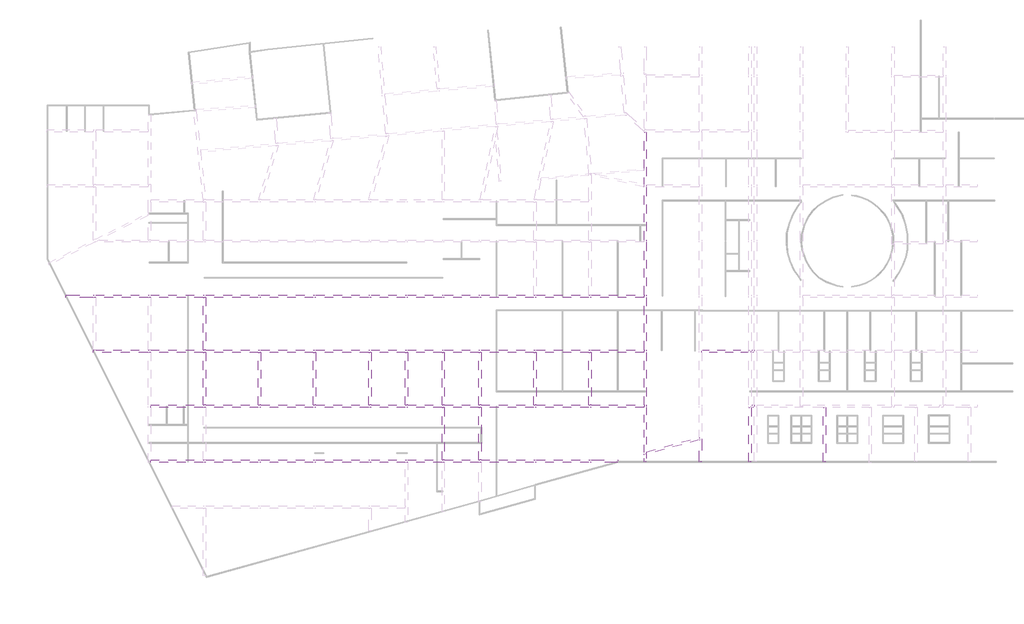
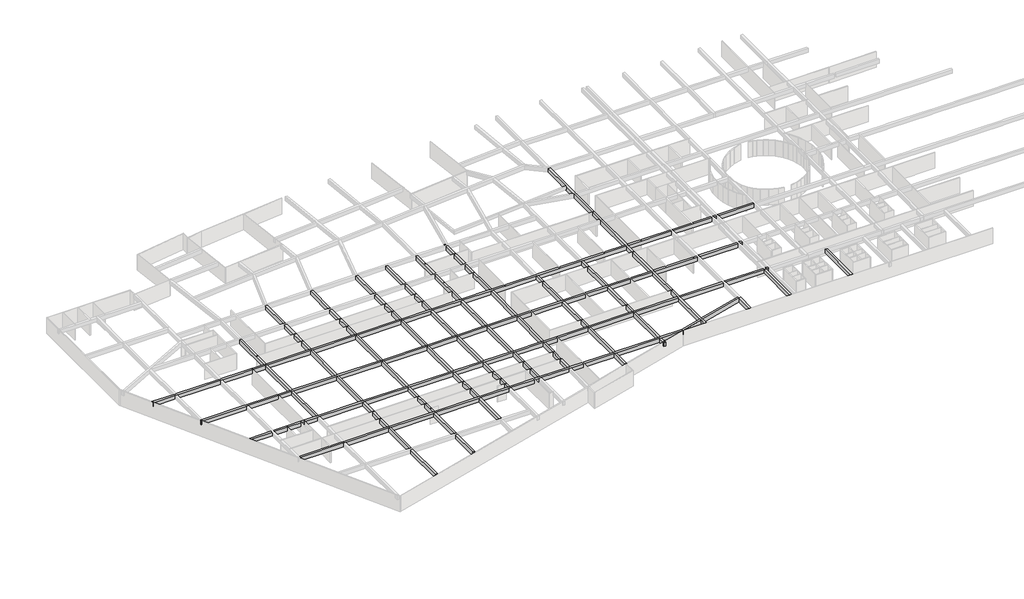
# One storey, part 5 of 8: 24 beams.
"""IFC4 building model written with IfcOpenShell, lengths in millimetres."""

from ifc_helpers import new_model, si_unit, frame, origin, place, context, project, spatial, polyline, outline, extrude, faceted_brep, element, save

model = new_model("IFC4")

# Units and contexts
model_context = context("Model", 3, world=origin())
ifc_project = project(units=[si_unit("LENGTHUNIT", "METRE", prefix="MILLI")], contexts=[model_context])

# Site, building, storey
site = spatial("IfcSite", under=ifc_project)
building = spatial("IfcBuilding", under=site)
storey = spatial("IfcBuildingStorey", under=building, Name="户型图", Elevation=0.0)

# Beams
placement = place(None, origin())
element("IfcBeam", 1, ObjectType="混凝土 - 矩形梁 : KL_beam", at=placement, inside=storey, context=model_context, shape_type="Brep", body=[
    faceted_brep([(397553.8653576, -29561.3735341, 3300.0), (397153.8653576, -29561.3735341, 3300.0), (397153.8653576, -29561.3735341, 2500.0), (397553.8653576, -29561.3735341, 2500.0), (397553.8653576, -28340.5712105, 3300.0), (397553.8653576, -27925.4258396, 3300.0), (397553.8653576, -20661.3735124, 3300.0), (397553.8653576, -20261.3735124, 3300.0), (397553.8653576, -11661.3735096, 3300.0), (397553.8653576, -11261.3735096, 3300.0), (397553.8653576, -2661.3735096, 3300.0), (397553.8653576, -2261.3735096, 3300.0), (397553.8653576, 6338.6264904, 3300.0), (397553.8653576, 6738.6264904, 3300.0), (397553.8653576, 15338.6264904, 3300.0), (397553.8653576, 15738.6264904, 3300.0), (397553.8653576, 24338.6264659, 3300.0), (397153.8653576, 24338.6264659, 3300.0), (397153.8653576, 18348.9010914, 3300.0), (397153.8653576, 18047.7660466, 3300.0), (397153.8653576, 15787.9497009, 3300.0), (397153.8653576, 15378.1921694, 3300.0), (397153.8653576, 6738.6264904, 3300.0), (397153.8653576, 6338.6264904, 3300.0), (397153.8653576, -2261.3735096, 3300.0), (397153.8653576, -2661.3735096, 3300.0), (397153.8653576, -11261.3735096, 3300.0), (397153.8653576, -11661.3735096, 3300.0), (397153.8653576, -20261.3735124, 3300.0), (397153.8653576, -20661.3735124, 3300.0), (397153.8653576, -28036.5369507, 3300.0), (397153.8653576, -28451.6823216, 3300.0), (397153.8653576, 24338.6264659, 2500.0), (397153.8653576, 15787.9497009, 2500.0), (397153.8653576, 15378.1921694, 2500.0), (397153.8653576, 6738.6264904, 2500.0), (397153.8653576, 6338.6264904, 2500.0), (397153.8653576, -2261.3735096, 2500.0), (397153.8653576, -2661.3735096, 2500.0), (397153.8653576, -11261.3735096, 2500.0), (397153.8653576, -11661.3735096, 2500.0), (397153.8653576, -20261.3735124, 2500.0), (397153.8653576, -20661.3735124, 2500.0), (397153.8653576, -28036.5369507, 2500.0), (397153.8653576, -28451.6823216, 2500.0), (397553.8653576, 24338.6264659, 2500.0), (397553.8653576, 15738.6264904, 2500.0), (397553.8653576, 15338.6264904, 2500.0), (397553.8653576, 6738.6264904, 2500.0), (397553.8653576, 6338.6264904, 2500.0), (397553.8653576, -2261.3735096, 2500.0), (397553.8653576, -2661.3735096, 2500.0), (397553.8653576, -11261.3735096, 2500.0), (397553.8653576, -11661.3735096, 2500.0), (397553.8653576, -20261.3735124, 2500.0), (397553.8653576, -20661.3735124, 2500.0), (397553.8653576, -27925.4258396, 2500.0), (397553.8653576, -28340.5712105, 2500.0)], [[[0, 1, 2, 3]], [[1, 0, 4, 5, 6, 7, 8, 9, 10, 11, 12, 13, 14, 15, 16, 17, 18, 19, 20, 21, 22, 23, 24, 25, 26, 27, 28, 29, 30, 31]], [[2, 1, 31, 30, 29, 28, 27, 26, 25, 24, 23, 22, 21, 20, 19, 18, 17, 32, 33, 34, 35, 36, 37, 38, 39, 40, 41, 42, 43, 44]], [[3, 2, 44, 43, 42, 41, 40, 39, 38, 37, 36, 35, 34, 33, 32, 45, 46, 47, 48, 49, 50, 51, 52, 53, 54, 55, 56, 57]], [[0, 3, 57, 56, 55, 54, 53, 52, 51, 50, 49, 48, 47, 46, 45, 16, 15, 14, 13, 12, 11, 10, 9, 8, 7, 6, 5, 4]], [[17, 16, 45, 32]]]),
])
element("IfcBeam", 2, ObjectType="混凝土 - 矩形梁 : KL_beam", at=placement, inside=storey, context=model_context, shape_type="Brep", body=[
    faceted_brep([(406153.8653576, -11661.3735096, 3300.0), (406153.8653576, -11261.3735096, 3300.0), (397553.8653576, -11261.3735096, 3300.0), (397553.8653576, -11661.3735096, 3300.0), (406153.8653576, -11261.3735096, 2500.0), (397553.8653576, -11261.3735096, 2500.0), (406153.8653576, -11661.3735096, 2500.0), (397553.8653576, -11661.3735096, 2500.0)], [[[0, 1, 2, 3]], [[1, 4, 5, 2]], [[4, 6, 7, 5]], [[6, 0, 3, 7]], [[1, 0, 6, 4]], [[3, 2, 5, 7]]]),
    faceted_brep([(397153.8653576, -11261.3735096, 3300.0), (397153.8653576, -11661.3735096, 3300.0), (397153.8653576, -11661.3735096, 2500.0), (397153.8653576, -11261.3735096, 2500.0), (307153.8653555, -11261.3735096, 3300.0), (307153.8653555, -11661.3735096, 3300.0), (316153.8653576, -11661.3735096, 3300.0), (316553.8653576, -11661.3735096, 3300.0), (325153.8653576, -11661.3735096, 3300.0), (325553.8653576, -11661.3735096, 3300.0), (334153.8653576, -11661.3735096, 3300.0), (334553.8653576, -11661.3735096, 3300.0), (343153.8653576, -11661.3735096, 3300.0), (343553.8653576, -11661.3735096, 3300.0), (352153.8653576, -11661.3735096, 3300.0), (352553.8653576, -11661.3735096, 3300.0), (358153.8653576, -11661.3735096, 3300.0), (358553.8653576, -11661.3735096, 3300.0), (364153.8653576, -11661.3735096, 3300.0), (364553.8653576, -11661.3735096, 3300.0), (370153.8653576, -11661.3735096, 3300.0), (370553.8653576, -11661.3735096, 3300.0), (379153.8653576, -11661.3735096, 3300.0), (379553.8653576, -11661.3735096, 3300.0), (388153.8653576, -11661.3735096, 3300.0), (388553.8653576, -11661.3735096, 3300.0), (388553.8653576, -11261.3735096, 3300.0), (388153.8653576, -11261.3735096, 3300.0), (379553.8653576, -11261.3735096, 3300.0), (379153.8653576, -11261.3735096, 3300.0), (370553.8653576, -11261.3735096, 3300.0), (370153.8653576, -11261.3735096, 3300.0), (364553.8653576, -11261.3735096, 3300.0), (364153.8653576, -11261.3735096, 3300.0), (358553.8653576, -11261.3735096, 3300.0), (358153.8653576, -11261.3735096, 3300.0), (352553.8653576, -11261.3735096, 3300.0), (352153.8653576, -11261.3735096, 3300.0), (343553.8653576, -11261.3735096, 3300.0), (343153.8653576, -11261.3735096, 3300.0), (334553.8653576, -11261.3735096, 3300.0), (334153.8653576, -11261.3735096, 3300.0), (325553.8653576, -11261.3735096, 3300.0), (325153.8653576, -11261.3735096, 3300.0), (316553.8653576, -11261.3735096, 3300.0), (316153.8653576, -11261.3735096, 3300.0), (307553.8653555, -11261.3735096, 3300.0), (307153.8653555, -11261.3735096, 2500.0), (388553.8653576, -11261.3735096, 2500.0), (388153.8653576, -11261.3735096, 2500.0), (379553.8653576, -11261.3735096, 2500.0), (379153.8653576, -11261.3735096, 2500.0), (370553.8653576, -11261.3735096, 2500.0), (370153.8653576, -11261.3735096, 2500.0), (364553.8653576, -11261.3735096, 2500.0), (364153.8653576, -11261.3735096, 2500.0), (358553.8653576, -11261.3735096, 2500.0), (358153.8653576, -11261.3735096, 2500.0), (352553.8653576, -11261.3735096, 2500.0), (352153.8653576, -11261.3735096, 2500.0), (343553.8653576, -11261.3735096, 2500.0), (343153.8653576, -11261.3735096, 2500.0), (334553.8653576, -11261.3735096, 2500.0), (334153.8653576, -11261.3735096, 2500.0), (325553.8653576, -11261.3735096, 2500.0), (325153.8653576, -11261.3735096, 2500.0), (316553.8653576, -11261.3735096, 2500.0), (316153.8653576, -11261.3735096, 2500.0), (307553.8653555, -11261.3735096, 2500.0), (307153.8653555, -11661.3735096, 2500.0), (388553.8653576, -11661.3735096, 2500.0), (388153.8653576, -11661.3735096, 2500.0), (379553.8653576, -11661.3735096, 2500.0), (379153.8653576, -11661.3735096, 2500.0), (370553.8653576, -11661.3735096, 2500.0), (370153.8653576, -11661.3735096, 2500.0), (364553.8653576, -11661.3735096, 2500.0), (364153.8653576, -11661.3735096, 2500.0), (358553.8653576, -11661.3735096, 2500.0), (358153.8653576, -11661.3735096, 2500.0), (352553.8653576, -11661.3735096, 2500.0), (352153.8653576, -11661.3735096, 2500.0), (343553.8653576, -11661.3735096, 2500.0), (343153.8653576, -11661.3735096, 2500.0), (334553.8653576, -11661.3735096, 2500.0), (334153.8653576, -11661.3735096, 2500.0), (325553.8653576, -11661.3735096, 2500.0), (325153.8653576, -11661.3735096, 2500.0), (316553.8653576, -11661.3735096, 2500.0), (316153.8653576, -11661.3735096, 2500.0)], [[[0, 1, 2, 3]], [[4, 5, 6, 7, 8, 9, 10, 11, 12, 13, 14, 15, 16, 17, 18, 19, 20, 21, 22, 23, 24, 25, 1, 0, 26, 27, 28, 29, 30, 31, 32, 33, 34, 35, 36, 37, 38, 39, 40, 41, 42, 43, 44, 45, 46]], [[47, 4, 46, 45, 44, 43, 42, 41, 40, 39, 38, 37, 36, 35, 34, 33, 32, 31, 30, 29, 28, 27, 26, 0, 3, 48, 49, 50, 51, 52, 53, 54, 55, 56, 57, 58, 59, 60, 61, 62, 63, 64, 65, 66, 67, 68]], [[69, 47, 68, 67, 66, 65, 64, 63, 62, 61, 60, 59, 58, 57, 56, 55, 54, 53, 52, 51, 50, 49, 48, 3, 2, 70, 71, 72, 73, 74, 75, 76, 77, 78, 79, 80, 81, 82, 83, 84, 85, 86, 87, 88, 89]], [[5, 69, 89, 88, 87, 86, 85, 84, 83, 82, 81, 80, 79, 78, 77, 76, 75, 74, 73, 72, 71, 70, 2, 1, 25, 24, 23, 22, 21, 20, 19, 18, 17, 16, 15, 14, 13, 12, 11, 10, 9, 8, 7, 6]], [[5, 4, 47, 69]]]),
])
element("IfcBeam", 3, ObjectType="混凝土 - 矩形梁 : KL_beam", at=placement, inside=storey, context=model_context, shape_type="Brep", body=[
    faceted_brep([(302728.8653513, -2261.3735096, 3300.0), (302728.8653513, -2261.3735096, 2500.0), (302728.8653513, -2661.3735096, 2500.0), (302728.8653513, -2661.3735096, 3300.0), (397153.8653576, -2261.3735096, 3300.0), (397153.8653576, -2661.3735096, 3300.0), (397153.8653576, -2661.3735096, 2500.0), (397153.8653576, -2261.3735096, 2500.0), (307153.8653555, -2661.3735096, 3300.0), (307553.8653555, -2661.3735096, 3300.0), (316153.8653576, -2661.3735096, 3300.0), (316553.8653576, -2661.3735096, 3300.0), (325153.8653576, -2661.3735096, 3300.0), (325553.8653576, -2661.3735096, 3300.0), (334153.8653576, -2661.3735096, 3300.0), (334553.8653576, -2661.3735096, 3300.0), (343153.8653576, -2661.3735096, 3300.0), (343553.8653576, -2661.3735096, 3300.0), (352153.8653576, -2661.3735096, 3300.0), (352553.8653576, -2661.3735096, 3300.0), (358153.8653576, -2661.3735096, 3300.0), (358553.8653576, -2661.3735096, 3300.0), (364153.8653576, -2661.3735096, 3300.0), (364553.8653576, -2661.3735096, 3300.0), (370153.8653576, -2661.3735096, 3300.0), (370553.8653576, -2661.3735096, 3300.0), (379153.8653576, -2661.3735096, 3300.0), (379553.8653576, -2661.3735096, 3300.0), (388153.8653576, -2661.3735096, 3300.0), (388553.8653576, -2661.3735096, 3300.0), (388553.8653576, -2261.3735096, 3300.0), (388153.8653576, -2261.3735096, 3300.0), (379553.8653576, -2261.3735096, 3300.0), (379153.8653576, -2261.3735096, 3300.0), (370553.8653576, -2261.3735096, 3300.0), (370153.8653576, -2261.3735096, 3300.0), (364553.8653576, -2261.3735096, 3300.0), (364153.8653576, -2261.3735096, 3300.0), (358553.8653576, -2261.3735096, 3300.0), (358153.8653576, -2261.3735096, 3300.0), (352553.8653576, -2261.3735096, 3300.0), (352153.8653576, -2261.3735096, 3300.0), (343553.8653576, -2261.3735096, 3300.0), (343153.8653576, -2261.3735096, 3300.0), (334553.8653576, -2261.3735096, 3300.0), (334153.8653576, -2261.3735096, 3300.0), (325553.8653576, -2261.3735096, 3300.0), (325153.8653576, -2261.3735096, 3300.0), (316553.8653576, -2261.3735096, 3300.0), (316153.8653576, -2261.3735096, 3300.0), (307553.8653555, -2261.3735096, 3300.0), (307153.8653555, -2261.3735096, 3300.0), (307153.8653555, -2661.3735096, 2500.0), (307553.8653555, -2661.3735096, 2500.0), (316153.8653576, -2661.3735096, 2500.0), (316553.8653576, -2661.3735096, 2500.0), (325153.8653576, -2661.3735096, 2500.0), (325553.8653576, -2661.3735096, 2500.0), (334153.8653576, -2661.3735096, 2500.0), (334553.8653576, -2661.3735096, 2500.0), (343153.8653576, -2661.3735096, 2500.0), (343553.8653576, -2661.3735096, 2500.0), (352153.8653576, -2661.3735096, 2500.0), (352553.8653576, -2661.3735096, 2500.0), (358153.8653576, -2661.3735096, 2500.0), (358553.8653576, -2661.3735096, 2500.0), (364153.8653576, -2661.3735096, 2500.0), (364553.8653576, -2661.3735096, 2500.0), (370153.8653576, -2661.3735096, 2500.0), (370553.8653576, -2661.3735096, 2500.0), (379153.8653576, -2661.3735096, 2500.0), (379553.8653576, -2661.3735096, 2500.0), (388153.8653576, -2661.3735096, 2500.0), (388553.8653576, -2661.3735096, 2500.0), (307153.8653555, -2261.3735096, 2500.0), (307553.8653555, -2261.3735096, 2500.0), (316153.8653576, -2261.3735096, 2500.0), (316553.8653576, -2261.3735096, 2500.0), (325153.8653576, -2261.3735096, 2500.0), (325553.8653576, -2261.3735096, 2500.0), (334153.8653576, -2261.3735096, 2500.0), (334553.8653576, -2261.3735096, 2500.0), (343153.8653576, -2261.3735096, 2500.0), (343553.8653576, -2261.3735096, 2500.0), (352153.8653576, -2261.3735096, 2500.0), (352553.8653576, -2261.3735096, 2500.0), (358153.8653576, -2261.3735096, 2500.0), (358553.8653576, -2261.3735096, 2500.0), (364153.8653576, -2261.3735096, 2500.0), (364553.8653576, -2261.3735096, 2500.0), (370153.8653576, -2261.3735096, 2500.0), (370553.8653576, -2261.3735096, 2500.0), (379153.8653576, -2261.3735096, 2500.0), (379553.8653576, -2261.3735096, 2500.0), (388153.8653576, -2261.3735096, 2500.0), (388553.8653576, -2261.3735096, 2500.0)], [[[0, 1, 2, 3]], [[4, 5, 6, 7]], [[0, 3, 8, 9, 10, 11, 12, 13, 14, 15, 16, 17, 18, 19, 20, 21, 22, 23, 24, 25, 26, 27, 28, 29, 5, 4, 30, 31, 32, 33, 34, 35, 36, 37, 38, 39, 40, 41, 42, 43, 44, 45, 46, 47, 48, 49, 50, 51]], [[3, 2, 52, 53, 54, 55, 56, 57, 58, 59, 60, 61, 62, 63, 64, 65, 66, 67, 68, 69, 70, 71, 72, 73, 6, 5, 29, 28, 27, 26, 25, 24, 23, 22, 21, 20, 19, 18, 17, 16, 15, 14, 13, 12, 11, 10, 9, 8]], [[2, 1, 74, 75, 76, 77, 78, 79, 80, 81, 82, 83, 84, 85, 86, 87, 88, 89, 90, 91, 92, 93, 94, 95, 7, 6, 73, 72, 71, 70, 69, 68, 67, 66, 65, 64, 63, 62, 61, 60, 59, 58, 57, 56, 55, 54, 53, 52]], [[1, 0, 51, 50, 49, 48, 47, 46, 45, 44, 43, 42, 41, 40, 39, 38, 37, 36, 35, 34, 33, 32, 31, 30, 4, 7, 95, 94, 93, 92, 91, 90, 89, 88, 87, 86, 85, 84, 83, 82, 81, 80, 79, 78, 77, 76, 75, 74]]]),
    faceted_brep([(422653.8653576, -2661.3735096, 3300.0), (422653.8653576, -2261.3735096, 3300.0), (415553.8653576, -2261.3735096, 3300.0), (415553.8653576, -2661.3735096, 3300.0), (422653.8653576, -2661.3735096, 2500.0), (415553.8653576, -2661.3735096, 2500.0), (422653.8653576, -2261.3735096, 2500.0), (415553.8653576, -2261.3735096, 2500.0)], [[[0, 1, 2, 3]], [[4, 0, 3, 5]], [[6, 4, 5, 7]], [[1, 6, 7, 2]], [[1, 0, 4, 6]], [[3, 2, 7, 5]]]),
    faceted_brep([(415153.8653576, -2261.3735096, 3300.0), (415153.8653576, -2661.3735096, 3300.0), (415153.8653576, -2661.3735096, 2500.0), (415153.8653576, -2261.3735096, 2500.0), (414653.8653576, -2261.3735096, 3300.0), (414653.8653576, -2661.3735096, 3300.0), (414653.8653576, -2661.3735096, 2500.0), (414653.8653576, -2261.3735096, 2500.0)], [[[0, 1, 2, 3]], [[1, 0, 4, 5]], [[2, 1, 5, 6]], [[3, 2, 6, 7]], [[0, 3, 7, 4]], [[5, 4, 7, 6]]]),
    faceted_brep([(414253.8653576, -2261.3735096, 3300.0), (414253.8653576, -2661.3735096, 3300.0), (414253.8653576, -2661.3735096, 2500.0), (414253.8653576, -2261.3735096, 2500.0), (406553.8653576, -2261.3735096, 3300.0), (406553.8653576, -2661.3735096, 3300.0), (406553.8653576, -2661.3735096, 2500.0), (406553.8653576, -2261.3735096, 2500.0)], [[[0, 1, 2, 3]], [[1, 0, 4, 5]], [[2, 1, 5, 6]], [[3, 2, 6, 7]], [[0, 3, 7, 4]], [[5, 4, 7, 6]]]),
    faceted_brep([(406153.8653576, -2261.3735096, 3300.0), (406153.8653576, -2661.3735096, 3300.0), (406153.8653576, -2661.3735096, 2500.0), (406153.8653576, -2261.3735096, 2500.0), (397553.8653576, -2261.3735096, 3300.0), (397553.8653576, -2661.3735096, 3300.0), (397553.8653576, -2661.3735096, 2500.0), (397553.8653576, -2261.3735096, 2500.0)], [[[0, 1, 2, 3]], [[1, 0, 4, 5]], [[2, 1, 5, 6]], [[3, 2, 6, 7]], [[0, 3, 7, 4]], [[5, 4, 7, 6]]]),
])
element("IfcBeam", 4, ObjectType="混凝土 - 矩形梁 : KL_beam", at=placement, inside=storey, context=model_context, shape_type="SweptSolid", body=[
    extrude(outline(polyline([(325153.8653576, 6338.6264904), (325553.8653576, 6338.6264904), (325553.8653576, -2261.3735096), (325153.8653576, -2261.3735096), (325153.8653576, 6338.6264904)])), frame((0.0, 0.0, 2500.0), z_axis=(0.0, 0.0, 1.0), x_axis=(1.0, 0.0, 0.0)), (0.0, 0.0, 1.0), 800.0),
    extrude(outline(polyline([(325553.8653576, -11261.3735096), (325153.8653576, -11261.3735096), (325153.8653576, -2661.3735096), (325553.8653576, -2661.3735096), (325553.8653576, -11261.3735096)])), frame((0.0, 0.0, 2500.0), z_axis=(0.0, 0.0, 1.0), x_axis=(1.0, 0.0, 0.0)), (0.0, 0.0, 1.0), 800.0),
])
element("IfcBeam", 5, ObjectType="混凝土 - 矩形梁 : KL_beam", at=placement, inside=storey, context=model_context, shape_type="Brep", body=[
    faceted_brep([(311853.8653587, -20261.3735124, 3300.0), (311853.8653587, -20261.3735124, 2500.0), (311853.8653587, -20661.3735124, 2500.0), (311853.8653587, -20661.3735124, 3300.0), (316153.8653576, -20261.3735124, 3300.0), (316153.8653576, -20661.3735124, 3300.0), (316153.8653576, -20661.3735124, 2500.0), (316153.8653576, -20261.3735124, 2500.0)], [[[0, 1, 2, 3]], [[4, 5, 6, 7]], [[0, 3, 5, 4]], [[3, 2, 6, 5]], [[2, 1, 7, 6]], [[1, 0, 4, 7]]]),
    faceted_brep([(414253.8653576, -20661.3735124, 3300.0), (414253.8653576, -20261.3735124, 3300.0), (406553.8653576, -20261.3735124, 3300.0), (406553.8653576, -20661.3735124, 3300.0), (414253.8653576, -20661.3735124, 2500.0), (406553.8653576, -20661.3735124, 2500.0), (414253.8653576, -20261.3735124, 2500.0), (406553.8653576, -20261.3735124, 2500.0)], [[[0, 1, 2, 3]], [[4, 0, 3, 5]], [[6, 4, 5, 7]], [[1, 6, 7, 2]], [[1, 0, 4, 6]], [[3, 2, 7, 5]]]),
    faceted_brep([(406153.8653576, -20261.3735124, 3300.0), (406153.8653576, -20661.3735124, 3300.0), (406153.8653576, -20661.3735124, 2500.0), (406153.8653576, -20261.3735124, 2500.0), (397553.8653576, -20261.3735124, 3300.0), (397553.8653576, -20661.3735124, 3300.0), (397553.8653576, -20661.3735124, 2500.0), (397553.8653576, -20261.3735124, 2500.0)], [[[0, 1, 2, 3]], [[1, 0, 4, 5]], [[2, 1, 5, 6]], [[3, 2, 6, 7]], [[0, 3, 7, 4]], [[5, 4, 7, 6]]]),
    faceted_brep([(397153.8653576, -20261.3735124, 3300.0), (397153.8653576, -20661.3735124, 3300.0), (397153.8653576, -20661.3735124, 2500.0), (397153.8653576, -20261.3735124, 2500.0), (388553.8653576, -20261.3735124, 3300.0), (388153.8653576, -20261.3735124, 3300.0), (379553.8653576, -20261.3735124, 3300.0), (379153.8653576, -20261.3735124, 3300.0), (370553.8653576, -20261.3735124, 3300.0), (370153.8653576, -20261.3735124, 3300.0), (364553.8653576, -20261.3735124, 3300.0), (364153.8653576, -20261.3735124, 3300.0), (358553.8653576, -20261.3735124, 3300.0), (358153.8653576, -20261.3735124, 3300.0), (352553.8653576, -20261.3735124, 3300.0), (352153.8653576, -20261.3735124, 3300.0), (343553.8653576, -20261.3735124, 3300.0), (343153.8653576, -20261.3735124, 3300.0), (334553.8653576, -20261.3735124, 3300.0), (334153.8653576, -20261.3735124, 3300.0), (325553.8653576, -20261.3735124, 3300.0), (325153.8653576, -20261.3735124, 3300.0), (316553.8653576, -20261.3735124, 3300.0), (316553.8653576, -20661.3735124, 3300.0), (325153.8653576, -20661.3735124, 3300.0), (325553.8653576, -20661.3735124, 3300.0), (334153.8653576, -20661.3735124, 3300.0), (334553.8653576, -20661.3735124, 3300.0), (343153.8653576, -20661.3735124, 3300.0), (343553.8653576, -20661.3735124, 3300.0), (352153.8653576, -20661.3735124, 3300.0), (352553.8653576, -20661.3735124, 3300.0), (358153.8653576, -20661.3735124, 3300.0), (358553.8653576, -20661.3735124, 3300.0), (364153.8653576, -20661.3735124, 3300.0), (364553.8653576, -20661.3735124, 3300.0), (370153.8653576, -20661.3735124, 3300.0), (370553.8653576, -20661.3735124, 3300.0), (379153.8653576, -20661.3735124, 3300.0), (379553.8653576, -20661.3735124, 3300.0), (388153.8653576, -20661.3735124, 3300.0), (388553.8653576, -20661.3735124, 3300.0), (316553.8653576, -20661.3735124, 2500.0), (325153.8653576, -20661.3735124, 2500.0), (325553.8653576, -20661.3735124, 2500.0), (334153.8653576, -20661.3735124, 2500.0), (334553.8653576, -20661.3735124, 2500.0), (343153.8653576, -20661.3735124, 2500.0), (343553.8653576, -20661.3735124, 2500.0), (352153.8653576, -20661.3735124, 2500.0), (352553.8653576, -20661.3735124, 2500.0), (358153.8653576, -20661.3735124, 2500.0), (358553.8653576, -20661.3735124, 2500.0), (364153.8653576, -20661.3735124, 2500.0), (364553.8653576, -20661.3735124, 2500.0), (370153.8653576, -20661.3735124, 2500.0), (370553.8653576, -20661.3735124, 2500.0), (379153.8653576, -20661.3735124, 2500.0), (379553.8653576, -20661.3735124, 2500.0), (388153.8653576, -20661.3735124, 2500.0), (388553.8653576, -20661.3735124, 2500.0), (316553.8653576, -20261.3735124, 2500.0), (325153.8653576, -20261.3735124, 2500.0), (325553.8653576, -20261.3735124, 2500.0), (334153.8653576, -20261.3735124, 2500.0), (334553.8653576, -20261.3735124, 2500.0), (343153.8653576, -20261.3735124, 2500.0), (343553.8653576, -20261.3735124, 2500.0), (352153.8653576, -20261.3735124, 2500.0), (352553.8653576, -20261.3735124, 2500.0), (358153.8653576, -20261.3735124, 2500.0), (358553.8653576, -20261.3735124, 2500.0), (364153.8653576, -20261.3735124, 2500.0), (364553.8653576, -20261.3735124, 2500.0), (370153.8653576, -20261.3735124, 2500.0), (370553.8653576, -20261.3735124, 2500.0), (379153.8653576, -20261.3735124, 2500.0), (379553.8653576, -20261.3735124, 2500.0), (388153.8653576, -20261.3735124, 2500.0), (388553.8653576, -20261.3735124, 2500.0)], [[[0, 1, 2, 3]], [[1, 0, 4, 5, 6, 7, 8, 9, 10, 11, 12, 13, 14, 15, 16, 17, 18, 19, 20, 21, 22, 23, 24, 25, 26, 27, 28, 29, 30, 31, 32, 33, 34, 35, 36, 37, 38, 39, 40, 41]], [[2, 1, 41, 40, 39, 38, 37, 36, 35, 34, 33, 32, 31, 30, 29, 28, 27, 26, 25, 24, 23, 42, 43, 44, 45, 46, 47, 48, 49, 50, 51, 52, 53, 54, 55, 56, 57, 58, 59, 60]], [[3, 2, 60, 59, 58, 57, 56, 55, 54, 53, 52, 51, 50, 49, 48, 47, 46, 45, 44, 43, 42, 61, 62, 63, 64, 65, 66, 67, 68, 69, 70, 71, 72, 73, 74, 75, 76, 77, 78, 79]], [[0, 3, 79, 78, 77, 76, 75, 74, 73, 72, 71, 70, 69, 68, 67, 66, 65, 64, 63, 62, 61, 22, 21, 20, 19, 18, 17, 16, 15, 14, 13, 12, 11, 10, 9, 8, 7, 6, 5, 4]], [[23, 22, 61, 42]]]),
])
element("IfcBeam", 6, ObjectType="混凝土 - 矩形梁 : KL_beam", at=placement, inside=storey, context=model_context, shape_type="SweptSolid", body=[
    extrude(outline(polyline([(414653.8653576, -29561.3735124), (414253.8653576, -29561.3735124), (414253.8653576, -20661.3735124), (414653.8653576, -20661.3735124), (414653.8653576, -29561.3735124)])), frame((0.0, 0.0, 2500.0), z_axis=(0.0, 0.0, 1.0), x_axis=(1.0, 0.0, 0.0)), (0.0, 0.0, 1.0), 800.0),
])
element("IfcBeam", 7, ObjectType="混凝土 - 矩形梁 : KL_beam", at=placement, inside=storey, context=model_context, shape_type="SweptSolid", body=[
    extrude(outline(polyline([(406553.8653576, -29567.6681706), (406153.8653576, -29567.6681706), (406153.8653576, -25951.6823221), (406553.8653576, -25840.571211), (406553.8653576, -29567.6681706)])), frame((0.0, 0.0, 2500.0), z_axis=(0.0, 0.0, 1.0), x_axis=(1.0, 0.0, 0.0)), (0.0, 0.0, 1.0), 800.0),
])
element("IfcBeam", 8, ObjectType="混凝土 - 矩形梁 : KL_beam", at=placement, inside=storey, context=model_context, shape_type="SweptSolid", body=[
    extrude(outline(polyline([(392891.8762903, -29635.5681734), (392837.3529549, -29235.5681734), (397153.8653576, -28036.5369507), (397153.8653576, -28451.6823216), (392891.8762903, -29635.5681734)])), frame((0.0, 0.0, 2500.0), z_axis=(0.0, 0.0, 1.0), x_axis=(1.0, 0.0, 0.0)), (0.0, 0.0, 1.0), 800.0),
    extrude(outline(polyline([(406153.8653576, -25536.5369512), (406153.8653576, -25951.6823221), (397553.8653576, -28340.5712105), (397553.8653576, -27925.4258396), (406153.8653576, -25536.5369512)])), frame((0.0, 0.0, 2500.0), z_axis=(0.0, 0.0, 1.0), x_axis=(1.0, 0.0, 0.0)), (0.0, 0.0, 1.0), 800.0),
])
element("IfcBeam", 9, ObjectType="混凝土 - 矩形梁 : KL_beam", at=placement, inside=storey, context=model_context, shape_type="Brep", body=[
    faceted_brep([(392891.8762903, -29635.5681734, 3300.0), (392837.3529549, -29235.5681734, 3300.0), (388553.8653576, -29235.5681734, 3300.0), (388153.8653576, -29235.5681734, 3300.0), (379553.8653576, -29235.5681734, 3300.0), (379153.8653576, -29235.5681734, 3300.0), (370553.8653576, -29235.5681734, 3300.0), (370153.8653576, -29235.5681734, 3300.0), (364553.8653576, -29235.5681734, 3300.0), (364153.8653576, -29235.5681734, 3300.0), (358553.8653576, -29235.5681734, 3300.0), (358153.8653576, -29235.5681734, 3300.0), (352553.8653576, -29235.5681734, 3300.0), (352153.8653576, -29235.5681734, 3300.0), (343553.8653576, -29235.5681734, 3300.0), (343153.8653576, -29235.5681734, 3300.0), (334553.8653576, -29235.5681734, 3300.0), (334153.8653576, -29235.5681734, 3300.0), (325553.8653576, -29235.5681734, 3300.0), (325153.8653576, -29235.5681734, 3300.0), (316553.8653576, -29235.5681734, 3300.0), (316553.8653576, -29635.5681734, 3300.0), (325153.8653576, -29635.5681734, 3300.0), (325553.8653576, -29635.5681734, 3300.0), (334153.8653576, -29635.5681734, 3300.0), (334553.8653576, -29635.5681734, 3300.0), (343153.8653576, -29635.5681734, 3300.0), (343553.8653576, -29635.5681734, 3300.0), (352153.8653576, -29635.5681734, 3300.0), (352553.8653576, -29635.5681734, 3300.0), (358153.8653576, -29635.5681734, 3300.0), (358553.8653576, -29635.5681734, 3300.0), (364153.8653576, -29635.5681734, 3300.0), (364553.8653576, -29635.5681734, 3300.0), (370153.8653576, -29635.5681734, 3300.0), (370553.8653576, -29635.5681734, 3300.0), (379153.8653576, -29635.5681734, 3300.0), (379553.8653576, -29635.5681734, 3300.0), (388153.8653576, -29635.5681734, 3300.0), (388553.8653576, -29635.5681734, 3300.0), (392837.3529549, -29235.5681734, 2500.0), (388553.8653576, -29235.5681734, 2500.0), (388153.8653576, -29235.5681734, 2500.0), (379553.8653576, -29235.5681734, 2500.0), (379153.8653576, -29235.5681734, 2500.0), (370553.8653576, -29235.5681734, 2500.0), (370153.8653576, -29235.5681734, 2500.0), (364553.8653576, -29235.5681734, 2500.0), (364153.8653576, -29235.5681734, 2500.0), (358553.8653576, -29235.5681734, 2500.0), (358153.8653576, -29235.5681734, 2500.0), (352553.8653576, -29235.5681734, 2500.0), (352153.8653576, -29235.5681734, 2500.0), (343553.8653576, -29235.5681734, 2500.0), (343153.8653576, -29235.5681734, 2500.0), (334553.8653576, -29235.5681734, 2500.0), (334153.8653576, -29235.5681734, 2500.0), (325553.8653576, -29235.5681734, 2500.0), (325153.8653576, -29235.5681734, 2500.0), (316553.8653576, -29235.5681734, 2500.0), (392891.8762903, -29635.5681734, 2500.0), (388553.8653576, -29635.5681734, 2500.0), (388153.8653576, -29635.5681734, 2500.0), (379553.8653576, -29635.5681734, 2500.0), (379153.8653576, -29635.5681734, 2500.0), (370553.8653576, -29635.5681734, 2500.0), (370153.8653576, -29635.5681734, 2500.0), (364553.8653576, -29635.5681734, 2500.0), (364153.8653576, -29635.5681734, 2500.0), (358553.8653576, -29635.5681734, 2500.0), (358153.8653576, -29635.5681734, 2500.0), (352553.8653576, -29635.5681734, 2500.0), (352153.8653576, -29635.5681734, 2500.0), (343553.8653576, -29635.5681734, 2500.0), (343153.8653576, -29635.5681734, 2500.0), (334553.8653576, -29635.5681734, 2500.0), (334153.8653576, -29635.5681734, 2500.0), (325553.8653576, -29635.5681734, 2500.0), (325153.8653576, -29635.5681734, 2500.0), (316553.8653576, -29635.5681734, 2500.0)], [[[0, 1, 2, 3, 4, 5, 6, 7, 8, 9, 10, 11, 12, 13, 14, 15, 16, 17, 18, 19, 20, 21, 22, 23, 24, 25, 26, 27, 28, 29, 30, 31, 32, 33, 34, 35, 36, 37, 38, 39]], [[1, 40, 41, 42, 43, 44, 45, 46, 47, 48, 49, 50, 51, 52, 53, 54, 55, 56, 57, 58, 59, 20, 19, 18, 17, 16, 15, 14, 13, 12, 11, 10, 9, 8, 7, 6, 5, 4, 3, 2]], [[40, 60, 61, 62, 63, 64, 65, 66, 67, 68, 69, 70, 71, 72, 73, 74, 75, 76, 77, 78, 79, 59, 58, 57, 56, 55, 54, 53, 52, 51, 50, 49, 48, 47, 46, 45, 44, 43, 42, 41]], [[60, 0, 39, 38, 37, 36, 35, 34, 33, 32, 31, 30, 29, 28, 27, 26, 25, 24, 23, 22, 21, 79, 78, 77, 76, 75, 74, 73, 72, 71, 70, 69, 68, 67, 66, 65, 64, 63, 62, 61]], [[0, 60, 40, 1]], [[21, 20, 59, 79]]]),
])
element("IfcBeam", 10, ObjectType="混凝土 - 矩形梁 : KL_beam", at=placement, inside=storey, context=model_context, shape_type="SweptSolid", body=[
    extrude(outline(polyline([(352553.8653576, -36750.8162358), (352153.8653576, -36750.8162358), (352153.8653576, -29635.5681734), (352553.8653576, -29635.5681734), (352553.8653576, -36750.8162358)])), frame((0.0, 0.0, 2500.0), z_axis=(0.0, 0.0, 1.0), x_axis=(1.0, 0.0, 0.0)), (0.0, 0.0, 1.0), 800.0),
    extrude(outline(polyline([(352153.8653576, 12938.6264904), (352553.8653576, 12938.6264904), (352553.8653576, 6738.6264904), (352153.8653576, 6738.6264904), (352153.8653576, 12938.6264904)])), frame((0.0, 0.0, 2500.0), z_axis=(0.0, 0.0, 1.0), x_axis=(1.0, 0.0, 0.0)), (0.0, 0.0, 1.0), 800.0),
    extrude(outline(polyline([(352553.8653576, -11261.3735096), (352153.8653576, -11261.3735096), (352153.8653576, -2661.3735096), (352553.8653576, -2661.3735096), (352553.8653576, -11261.3735096)])), frame((0.0, 0.0, 2500.0), z_axis=(0.0, 0.0, 1.0), x_axis=(1.0, 0.0, 0.0)), (0.0, 0.0, 1.0), 800.0),
    extrude(outline(polyline([(352153.8653576, -11661.3735096), (352553.8653576, -11661.3735096), (352553.8653576, -20261.3735124), (352153.8653576, -20261.3735124), (352153.8653576, -11661.3735096)])), frame((0.0, 0.0, 2500.0), z_axis=(0.0, 0.0, 1.0), x_axis=(1.0, 0.0, 0.0)), (0.0, 0.0, 1.0), 800.0),
    extrude(outline(polyline([(352553.8653576, -2261.3735096), (352153.8653576, -2261.3735096), (352153.8653576, 6338.6264904), (352553.8653576, 6338.6264904), (352553.8653576, -2261.3735096)])), frame((0.0, 0.0, 2500.0), z_axis=(0.0, 0.0, 1.0), x_axis=(1.0, 0.0, 0.0)), (0.0, 0.0, 1.0), 800.0),
    extrude(outline(polyline([(352153.8653576, -20661.3735124), (352553.8653576, -20661.3735124), (352553.8653576, -29235.5681734), (352153.8653576, -29235.5681734), (352153.8653576, -20661.3735124)])), frame((0.0, 0.0, 2500.0), z_axis=(0.0, 0.0, 1.0), x_axis=(1.0, 0.0, 0.0)), (0.0, 0.0, 1.0), 800.0),
])
element("IfcBeam", 11, ObjectType="混凝土 - 矩形梁 : KL_beam", at=placement, inside=storey, context=model_context, shape_type="SweptSolid", body=[
    extrude(outline(polyline([(343553.8653576, -43188.4637935), (343153.8653576, -43188.4637935), (343153.8653576, -37150.8162358), (343553.8653576, -37150.8162358), (343553.8653576, -43188.4637935)])), frame((0.0, 0.0, 2500.0), z_axis=(0.0, 0.0, 1.0), x_axis=(1.0, 0.0, 0.0)), (0.0, 0.0, 1.0), 800.0),
    extrude(outline(polyline([(343153.8653576, 12938.6264904), (343553.8653576, 12938.6264904), (343553.8653576, 6738.6264904), (343153.8653576, 6738.6264904), (343153.8653576, 12938.6264904)])), frame((0.0, 0.0, 2500.0), z_axis=(0.0, 0.0, 1.0), x_axis=(1.0, 0.0, 0.0)), (0.0, 0.0, 1.0), 800.0),
    extrude(outline(polyline([(343553.8653576, -11261.3735096), (343153.8653576, -11261.3735096), (343153.8653576, -2661.3735096), (343553.8653576, -2661.3735096), (343553.8653576, -11261.3735096)])), frame((0.0, 0.0, 2500.0), z_axis=(0.0, 0.0, 1.0), x_axis=(1.0, 0.0, 0.0)), (0.0, 0.0, 1.0), 800.0),
    extrude(outline(polyline([(343153.8653576, -11661.3735096), (343553.8653576, -11661.3735096), (343553.8653576, -20261.3735124), (343153.8653576, -20261.3735124), (343153.8653576, -11661.3735096)])), frame((0.0, 0.0, 2500.0), z_axis=(0.0, 0.0, 1.0), x_axis=(1.0, 0.0, 0.0)), (0.0, 0.0, 1.0), 800.0),
    extrude(outline(polyline([(343553.8653576, -2261.3735096), (343153.8653576, -2261.3735096), (343153.8653576, 6338.6264904), (343553.8653576, 6338.6264904), (343553.8653576, -2261.3735096)])), frame((0.0, 0.0, 2500.0), z_axis=(0.0, 0.0, 1.0), x_axis=(1.0, 0.0, 0.0)), (0.0, 0.0, 1.0), 800.0),
    extrude(outline(polyline([(343153.8653576, -20661.3735124), (343553.8653576, -20661.3735124), (343553.8653576, -29235.5681734), (343153.8653576, -29235.5681734), (343153.8653576, -20661.3735124)])), frame((0.0, 0.0, 2500.0), z_axis=(0.0, 0.0, 1.0), x_axis=(1.0, 0.0, 0.0)), (0.0, 0.0, 1.0), 800.0),
    extrude(outline(polyline([(343153.8653576, -29635.5681734), (343553.8653576, -29635.5681734), (343553.8653576, -36750.8162358), (343153.8653576, -36750.8162358), (343153.8653576, -29635.5681734)])), frame((0.0, 0.0, 2500.0), z_axis=(0.0, 0.0, 1.0), x_axis=(1.0, 0.0, 0.0)), (0.0, 0.0, 1.0), 800.0),
])
element("IfcBeam", 12, ObjectType="混凝土 - 矩形梁 : KL_beam", at=placement, inside=storey, context=model_context, shape_type="SweptSolid", body=[
    extrude(outline(polyline([(334553.8653576, -45688.4637932), (334153.8653576, -45688.4637932), (334153.8653576, -37150.8162358), (334553.8653576, -37150.8162358), (334553.8653576, -45688.4637932)])), frame((0.0, 0.0, 2500.0), z_axis=(0.0, 0.0, 1.0), x_axis=(1.0, 0.0, 0.0)), (0.0, 0.0, 1.0), 800.0),
    extrude(outline(polyline([(334553.8653576, -11261.3735096), (334153.8653576, -11261.3735096), (334153.8653576, -2661.3735096), (334553.8653576, -2661.3735096), (334553.8653576, -11261.3735096)])), frame((0.0, 0.0, 2500.0), z_axis=(0.0, 0.0, 1.0), x_axis=(1.0, 0.0, 0.0)), (0.0, 0.0, 1.0), 800.0),
    extrude(outline(polyline([(334153.8653576, 12938.6264904), (334553.8653576, 12938.6264904), (334553.8653576, 6738.6264904), (334153.8653576, 6738.6264904), (334153.8653576, 12938.6264904)])), frame((0.0, 0.0, 2500.0), z_axis=(0.0, 0.0, 1.0), x_axis=(1.0, 0.0, 0.0)), (0.0, 0.0, 1.0), 800.0),
    extrude(outline(polyline([(334153.8653576, -11661.3735096), (334553.8653576, -11661.3735096), (334553.8653576, -20261.3735124), (334153.8653576, -20261.3735124), (334153.8653576, -11661.3735096)])), frame((0.0, 0.0, 2500.0), z_axis=(0.0, 0.0, 1.0), x_axis=(1.0, 0.0, 0.0)), (0.0, 0.0, 1.0), 800.0),
    extrude(outline(polyline([(334553.8653576, -2261.3735096), (334153.8653576, -2261.3735096), (334153.8653576, 6338.6264904), (334553.8653576, 6338.6264904), (334553.8653576, -2261.3735096)])), frame((0.0, 0.0, 2500.0), z_axis=(0.0, 0.0, 1.0), x_axis=(1.0, 0.0, 0.0)), (0.0, 0.0, 1.0), 800.0),
    extrude(outline(polyline([(334153.8653576, -20661.3735124), (334553.8653576, -20661.3735124), (334553.8653576, -29235.5681734), (334153.8653576, -29235.5681734), (334153.8653576, -20661.3735124)])), frame((0.0, 0.0, 2500.0), z_axis=(0.0, 0.0, 1.0), x_axis=(1.0, 0.0, 0.0)), (0.0, 0.0, 1.0), 800.0),
    extrude(outline(polyline([(334153.8653576, -29635.5681734), (334553.8653576, -29635.5681734), (334553.8653576, -36750.8162358), (334153.8653576, -36750.8162358), (334153.8653576, -29635.5681734)])), frame((0.0, 0.0, 2500.0), z_axis=(0.0, 0.0, 1.0), x_axis=(1.0, 0.0, 0.0)), (0.0, 0.0, 1.0), 800.0),
])
element("IfcBeam", 13, ObjectType="混凝土 - 矩形梁 : KL_beam", at=placement, inside=storey, context=model_context, shape_type="SweptSolid", body=[
    extrude(outline(polyline([(414653.8653576, -20661.3735096), (414653.8653576, -20261.3735096), (415153.8653576, -20261.3735096), (415153.8653576, -20661.3735096), (414653.8653576, -20661.3735096)])), frame((0.0, 0.0, 2500.0), z_axis=(0.0, 0.0, 1.0), x_axis=(1.0, 0.0, 0.0)), (0.0, 0.0, 1.0), 800.0),
])
element("IfcBeam", 14, ObjectType="混凝土 - 矩形梁 : KL_beam", at=placement, inside=storey, context=model_context, shape_type="SweptSolid", body=[
    extrude(outline(polyline([(415153.8653576, -11261.3735096), (415153.8653576, -11661.3735096), (414653.8653576, -11661.3735096), (414653.8653576, -11261.3735096), (415153.8653576, -11261.3735096)])), frame((0.0, 0.0, 2500.0), z_axis=(0.0, 0.0, 1.0), x_axis=(1.0, 0.0, 0.0)), (0.0, 0.0, 1.0), 800.0),
])
element("IfcBeam", 15, ObjectType="混凝土 - 矩形梁 : KL_beam", at=placement, inside=storey, context=model_context, shape_type="SweptSolid", body=[
    extrude(outline(polyline([(414253.8653576, -11261.3735096), (414253.8653576, -11661.3735096), (406553.8653576, -11661.3735096), (406553.8653576, -11261.3735096), (414253.8653576, -11261.3735096)])), frame((0.0, 0.0, 2500.0), z_axis=(0.0, 0.0, 1.0), x_axis=(1.0, 0.0, 0.0)), (0.0, 0.0, 1.0), 800.0),
])
element("IfcBeam", 16, ObjectType="混凝土 - 矩形梁 : KL_beam", at=placement, inside=storey, context=model_context, shape_type="SweptSolid", body=[
    extrude(outline(polyline([(426803.8653576, -29561.3735096), (426403.8653576, -29561.3735096), (426403.8653576, -20661.3735096), (426803.8653576, -20661.3735096), (426803.8653576, -29561.3735096)])), frame((0.0, 0.0, 2500.0), z_axis=(0.0, 0.0, 1.0), x_axis=(1.0, 0.0, 0.0)), (0.0, 0.0, 1.0), 800.0),
])
element("IfcBeam", 17, ObjectType="混凝土 - 矩形梁 : KL_beam", at=placement, inside=storey, context=model_context, shape_type="SweptSolid", body=[
    extrude(outline(polyline([(370153.8653576, -20661.3735124), (370553.8653576, -20661.3735124), (370553.8653576, -29235.5681734), (370153.8653576, -29235.5681734), (370153.8653576, -20661.3735124)])), frame((0.0, 0.0, 2500.0), z_axis=(0.0, 0.0, 1.0), x_axis=(1.0, 0.0, 0.0)), (0.0, 0.0, 1.0), 800.0),
])
element("IfcBeam", 18, ObjectType="混凝土 - 矩形梁 : KL_beam", at=placement, inside=storey, context=model_context, shape_type="SweptSolid", body=[
    extrude(outline(polyline([(364153.8653576, -20661.3735124), (364553.8653576, -20661.3735124), (364553.8653576, -29235.5681734), (364153.8653576, -29235.5681734), (364153.8653576, -20661.3735124)])), frame((0.0, 0.0, 2500.0), z_axis=(0.0, 0.0, 1.0), x_axis=(1.0, 0.0, 0.0)), (0.0, 0.0, 1.0), 800.0),
])
element("IfcBeam", 19, ObjectType="混凝土 - 矩形梁 : KL_beam", at=placement, inside=storey, context=model_context, shape_type="SweptSolid", body=[
    extrude(outline(polyline([(358553.8653576, -29235.5681734), (358153.8653576, -29235.5681734), (358153.8653576, -20661.3735124), (358553.8653576, -20661.3735124), (358553.8653576, -29235.5681734)])), frame((0.0, 0.0, 2500.0), z_axis=(0.0, 0.0, 1.0), x_axis=(1.0, 0.0, 0.0)), (0.0, 0.0, 1.0), 800.0),
    extrude(outline(polyline([(358153.8653576, 12938.6264904), (358553.8653576, 12938.6264904), (358553.8653576, 6738.6264904), (358153.8653576, 6738.6264904), (358153.8653576, 12938.6264904)])), frame((0.0, 0.0, 2500.0), z_axis=(0.0, 0.0, 1.0), x_axis=(1.0, 0.0, 0.0)), (0.0, 0.0, 1.0), 800.0),
    extrude(outline(polyline([(358553.8653576, -11261.3735096), (358153.8653576, -11261.3735096), (358153.8653576, -2661.3735096), (358553.8653576, -2661.3735096), (358553.8653576, -11261.3735096)])), frame((0.0, 0.0, 2500.0), z_axis=(0.0, 0.0, 1.0), x_axis=(1.0, 0.0, 0.0)), (0.0, 0.0, 1.0), 800.0),
    extrude(outline(polyline([(358153.8653576, -11661.3735096), (358553.8653576, -11661.3735096), (358553.8653576, -20261.3735124), (358153.8653576, -20261.3735124), (358153.8653576, -11661.3735096)])), frame((0.0, 0.0, 2500.0), z_axis=(0.0, 0.0, 1.0), x_axis=(1.0, 0.0, 0.0)), (0.0, 0.0, 1.0), 800.0),
    extrude(outline(polyline([(358553.8653576, -2261.3735096), (358153.8653576, -2261.3735096), (358153.8653576, 6338.6264904), (358553.8653576, 6338.6264904), (358553.8653576, -2261.3735096)])), frame((0.0, 0.0, 2500.0), z_axis=(0.0, 0.0, 1.0), x_axis=(1.0, 0.0, 0.0)), (0.0, 0.0, 1.0), 800.0),
])
element("IfcBeam", 20, ObjectType="混凝土 - 矩形梁 : KL_beam", at=placement, inside=storey, context=model_context, shape_type="SweptSolid", body=[
    extrude(outline(polyline([(364553.8653576, -20261.3735124), (364153.8653576, -20261.3735124), (364153.8653576, -11661.3735096), (364553.8653576, -11661.3735096), (364553.8653576, -20261.3735124)])), frame((0.0, 0.0, 2500.0), z_axis=(0.0, 0.0, 1.0), x_axis=(1.0, 0.0, 0.0)), (0.0, 0.0, 1.0), 800.0),
    extrude(outline(polyline([(364153.8653576, 12938.6264904), (364553.8653576, 12938.6264904), (364553.8653576, 6738.6264904), (364153.8653576, 6738.6264904), (364153.8653576, 12938.6264904)])), frame((0.0, 0.0, 2500.0), z_axis=(0.0, 0.0, 1.0), x_axis=(1.0, 0.0, 0.0)), (0.0, 0.0, 1.0), 800.0),
    extrude(outline(polyline([(364553.8653576, -11261.3735096), (364153.8653576, -11261.3735096), (364153.8653576, -2661.3735096), (364553.8653576, -2661.3735096), (364553.8653576, -11261.3735096)])), frame((0.0, 0.0, 2500.0), z_axis=(0.0, 0.0, 1.0), x_axis=(1.0, 0.0, 0.0)), (0.0, 0.0, 1.0), 800.0),
    extrude(outline(polyline([(364553.8653576, -2261.3735096), (364153.8653576, -2261.3735096), (364153.8653576, 6338.6264904), (364553.8653576, 6338.6264904), (364553.8653576, -2261.3735096)])), frame((0.0, 0.0, 2500.0), z_axis=(0.0, 0.0, 1.0), x_axis=(1.0, 0.0, 0.0)), (0.0, 0.0, 1.0), 800.0),
])
element("IfcBeam", 21, ObjectType="混凝土 - 矩形梁 : KL_beam", at=placement, inside=storey, context=model_context, shape_type="Brep", body=[
    faceted_brep([(370153.8653576, 13438.6264857, 2500.0), (370153.8653576, 13438.6264857, 3300.0), (370411.6081056, 13438.6264857, 3300.0), (370411.6081056, 13438.6264857, 2500.0), (370153.8653576, 13338.6264904, 3300.0), (370390.9533063, 13338.6264904, 3300.0), (370153.8653576, 13338.6264904, 2500.0), (370390.9533063, 13338.6264904, 2500.0)], [[[0, 1, 2, 3]], [[1, 4, 5, 2]], [[6, 0, 3, 7]], [[1, 0, 6, 4]], [[4, 6, 7, 5]], [[3, 2, 5, 7]]]),
    faceted_brep([(370553.8653576, -20261.3735124, 3300.0), (370153.8653576, -20261.3735124, 3300.0), (370153.8653576, -20261.3735124, 2500.0), (370553.8653576, -20261.3735124, 2500.0), (370153.8653576, -11661.3735096, 3300.0), (370553.8653576, -11661.3735096, 3300.0), (370553.8653576, -11661.3735096, 2500.0), (370153.8653576, -11661.3735096, 2500.0)], [[[0, 1, 2, 3]], [[4, 5, 6, 7]], [[1, 0, 5, 4]], [[0, 3, 6, 5]], [[3, 2, 7, 6]], [[2, 1, 4, 7]]]),
    faceted_brep([(370553.8653576, -11261.3735096, 3300.0), (370153.8653576, -11261.3735096, 3300.0), (370153.8653576, -11261.3735096, 2500.0), (370553.8653576, -11261.3735096, 2500.0), (370153.8653576, -2661.3735096, 3300.0), (370553.8653576, -2661.3735096, 3300.0), (370553.8653576, -2661.3735096, 2500.0), (370153.8653576, -2661.3735096, 2500.0)], [[[0, 1, 2, 3]], [[4, 5, 6, 7]], [[1, 0, 5, 4]], [[0, 3, 6, 5]], [[3, 2, 7, 6]], [[2, 1, 4, 7]]]),
    faceted_brep([(370553.8653576, -2261.3735096, 3300.0), (370153.8653576, -2261.3735096, 3300.0), (370153.8653576, -2261.3735096, 2500.0), (370553.8653576, -2261.3735096, 2500.0), (370153.8653576, 6338.6264904, 3300.0), (370553.8653576, 6338.6264904, 3300.0), (370553.8653576, 6338.6264904, 2500.0), (370153.8653576, 6338.6264904, 2500.0)], [[[0, 1, 2, 3]], [[4, 5, 6, 7]], [[1, 0, 5, 4]], [[0, 3, 6, 5]], [[3, 2, 7, 6]], [[2, 1, 4, 7]]]),
    faceted_brep([(370553.8653576, 6738.6264904, 3300.0), (370153.8653576, 6738.6264904, 3300.0), (370153.8653576, 6738.6264904, 2500.0), (370553.8653576, 6738.6264904, 2500.0), (370553.8653576, 12938.6264904, 3300.0), (370553.8653576, 12938.6264904, 2500.0), (370308.3341052, 12938.6264904, 2500.0), (370153.8653576, 12938.6264904, 2500.0), (370153.8653576, 12938.6264904, 3300.0), (370308.3341052, 12938.6264904, 3300.0)], [[[0, 1, 2, 3]], [[4, 5, 6, 7, 8, 9]], [[1, 0, 4, 9, 8]], [[0, 3, 5, 4]], [[3, 2, 7, 6, 5]], [[2, 1, 8, 7]]]),
])
element("IfcBeam", 22, ObjectType="混凝土 - 矩形梁 : KL_beam", at=placement, inside=storey, context=model_context, shape_type="SweptSolid", body=[
    extrude(outline(polyline([(379553.8653576, -33335.5889547), (379153.8653576, -33335.5889547), (379153.8653576, -29635.5681734), (379553.8653576, -29635.5681734), (379553.8653576, -33335.5889547)])), frame((0.0, 0.0, 2500.0), z_axis=(0.0, 0.0, 1.0), x_axis=(1.0, 0.0, 0.0)), (0.0, 0.0, 1.0), 800.0),
    extrude(outline(polyline([(379153.8653576, -2661.3735096), (379553.8653576, -2661.3735096), (379553.8653576, -11261.3735096), (379153.8653576, -11261.3735096), (379153.8653576, -2661.3735096)])), frame((0.0, 0.0, 2500.0), z_axis=(0.0, 0.0, 1.0), x_axis=(1.0, 0.0, 0.0)), (0.0, 0.0, 1.0), 800.0),
    extrude(outline(polyline([(379153.8653576, -11661.3735096), (379553.8653576, -11661.3735096), (379553.8653576, -20261.3735124), (379153.8653576, -20261.3735124), (379153.8653576, -11661.3735096)])), frame((0.0, 0.0, 2500.0), z_axis=(0.0, 0.0, 1.0), x_axis=(1.0, 0.0, 0.0)), (0.0, 0.0, 1.0), 800.0),
    extrude(outline(polyline([(379153.8653576, -20661.3735124), (379553.8653576, -20661.3735124), (379553.8653576, -29235.5681734), (379153.8653576, -29235.5681734), (379153.8653576, -20661.3735124)])), frame((0.0, 0.0, 2500.0), z_axis=(0.0, 0.0, 1.0), x_axis=(1.0, 0.0, 0.0)), (0.0, 0.0, 1.0), 800.0),
])
element("IfcBeam", 23, ObjectType="混凝土 - 矩形梁 : KL_beam", at=placement, inside=storey, context=model_context, shape_type="SweptSolid", body=[
    extrude(outline(polyline([(388553.8653576, -31103.5364803), (388153.8653576, -31103.5364803), (388153.8653576, -29635.5681734), (388553.8653576, -29635.5681734), (388553.8653576, -31103.5364803)])), frame((0.0, 0.0, 2500.0), z_axis=(0.0, 0.0, 1.0), x_axis=(1.0, 0.0, 0.0)), (0.0, 0.0, 1.0), 800.0),
    extrude(outline(polyline([(388153.8653576, -2661.3735096), (388553.8653576, -2661.3735096), (388553.8653576, -11261.3735096), (388153.8653576, -11261.3735096), (388153.8653576, -2661.3735096)])), frame((0.0, 0.0, 2500.0), z_axis=(0.0, 0.0, 1.0), x_axis=(1.0, 0.0, 0.0)), (0.0, 0.0, 1.0), 800.0),
    extrude(outline(polyline([(388153.8653576, -11661.3735096), (388553.8653576, -11661.3735096), (388553.8653576, -20261.3735124), (388153.8653576, -20261.3735124), (388153.8653576, -11661.3735096)])), frame((0.0, 0.0, 2500.0), z_axis=(0.0, 0.0, 1.0), x_axis=(1.0, 0.0, 0.0)), (0.0, 0.0, 1.0), 800.0),
    extrude(outline(polyline([(388153.8653576, -20661.3735124), (388553.8653576, -20661.3735124), (388553.8653576, -29235.5681734), (388153.8653576, -29235.5681734), (388153.8653576, -20661.3735124)])), frame((0.0, 0.0, 2500.0), z_axis=(0.0, 0.0, 1.0), x_axis=(1.0, 0.0, 0.0)), (0.0, 0.0, 1.0), 800.0),
])
element("IfcBeam", 24, ObjectType="混凝土 - 矩形梁 : KL_beam", at=placement, inside=storey, context=model_context, shape_type="SweptSolid", body=[
    extrude(outline(polyline([(325153.8653576, -11661.3735096), (325553.8653576, -11661.3735096), (325553.8653576, -20261.3735124), (325153.8653576, -20261.3735124), (325153.8653576, -11661.3735096)])), frame((0.0, 0.0, 2500.0), z_axis=(0.0, 0.0, 1.0), x_axis=(1.0, 0.0, 0.0)), (0.0, 0.0, 1.0), 800.0),
])

save(model, "model.ifc")

# Revit data of these elements
# Type "混凝土 - 矩形梁 : KL_beam"
#   Length [instance default] = 1524 mm
#   b = 400 mm
#   h = 800 mm
#   Structural Material [instance default] = 混凝土 - 现场浇注混凝土
#   Assembly Code = ""
# Elements 1, 2, 3, 4, 5, 6, 7, 8, 9, 10, 11, 12, 13, 14, 15, 16, 17, 18, 19, 20, 21, 22, 23, 24 (IfcBeam, "混凝土 - 矩形梁 : KL_beam")
#   Comments = ""
#   Structural Material = none
#   Phase Created = 新构造
# Materials
#   "混凝土 - 现场浇注混凝土": class "混凝土", colour RGB 192 192 192, transparency 0
